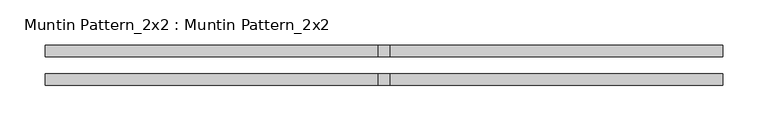
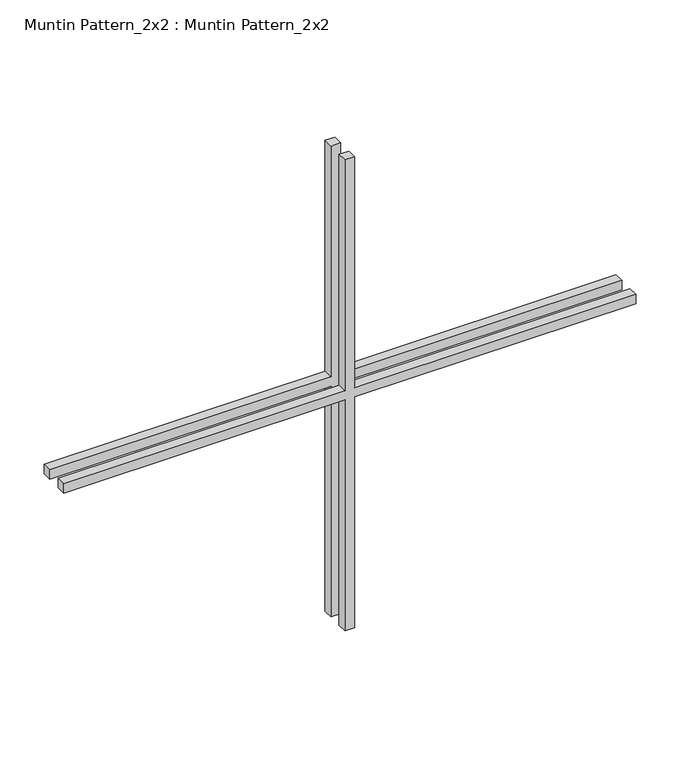
"""IFC4 building model written with IfcOpenShell, lengths in millimetres: proxy geometry, Muntin Pattern_2x2 : Muntin Pattern_2x2."""

from ifc_helpers import new_model, si_unit, frame, origin, place, context, project, spatial, polyline, outline, extrude, source, transform, mapped, element, save


def muntin_pattern_2x2_muntin_pattern_2x2_4af12bc4(model_context):
    return source(origin(), model_context, "Body", "SweptSolid", [
        extrude(outline(polyline([(332.1375, -6.35), (332.1375, -374.59375), (319.4375, -374.59375), (319.4375, -6.35), (0.0, -6.35), (0.0, 6.35), (319.4375, 6.35), (319.4375, 374.59375), (332.1375, 374.59375), (332.1375, 6.35), (651.575, 6.35), (651.575, -6.35), (332.1375, -6.35)])), frame((0.0, -22.225, 0.0), z_axis=(0.0, 1.0, 0.0), x_axis=(0.0, 0.0, 1.0)), (0.0, 0.0, 1.0), 12.7),
        extrude(outline(polyline([(332.1375, -6.35), (332.1375, -374.59375), (319.4375, -374.59375), (319.4375, -6.35), (0.0, -6.35), (0.0, 6.35), (319.4375, 6.35), (319.4375, 374.59375), (332.1375, 374.59375), (332.1375, 6.35), (651.575, 6.35), (651.575, -6.35), (332.1375, -6.35)])), frame((0.0, 9.525, 0.0), z_axis=(0.0, 1.0, 0.0), x_axis=(0.0, 0.0, 1.0)), (0.0, 0.0, 1.0), 12.7),
    ])


if __name__ == "__main__":
    model = new_model("IFC4")
    model_context = context("Model", 3, world=origin())
    ifc_project = project(units=[si_unit("LENGTHUNIT", "METRE", prefix="MILLI")], contexts=[model_context])
    site = spatial("IfcSite", under=ifc_project)
    building = spatial("IfcBuilding", under=site)
    placement = place(None, origin())
    muntin_pattern_2x2_muntin_pattern_2x2_shape = muntin_pattern_2x2_muntin_pattern_2x2_4af12bc4(model_context)
    element("IfcBuildingElementProxy", 1, Name="Muntin Pattern_2x2 : Muntin Pattern_2x2", ObjectType="Muntin Pattern_2x2 : Muntin Pattern_2x2", at=placement, inside=building, context=model_context, shape_type="MappedRepresentation", body=[
        mapped(muntin_pattern_2x2_muntin_pattern_2x2_shape, transform((0.0, 0.0, 0.0), x_axis=(1.0, 0.0, 0.0), y_axis=(0.0, 1.0, 0.0), z_axis=(0.0, 0.0, 1.0))),
    ])
    save(model, "model.ifc")

# Revit data of these elements
# Type "Muntin Pattern_2x2 : Muntin Pattern_2x2"
#   Width [instance default] = 121.92 cm
#   Thickness = 1.27 cm
#   Height [instance default] = 121.92 cm
#   Distance = 1.905 cm
#   Interior Material [instance default] = none
#   Exterior Material [instance default] = none
# Element 1 (IfcBuildingElementProxy, "Muntin Pattern_2x2 : Muntin Pattern_2x2")
#   Width = 74.9188 cm
#   Height = 65.1575 cm
#   Interior Material = Wood - Stained
#   Exterior Material = Clad - White
#   Materials on its faces: "Clad - White", "Wood - Stained"
# Materials
#   "Clad - White": class "Wood", colour RGB 242 242 238, transparency 0, Cost = 0
#   "Wood - Stained": class "Wood", colour RGB 224 178 126, transparency 0, Cost = 0
